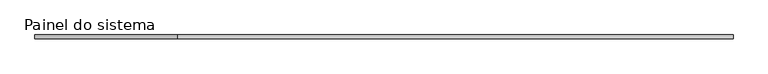
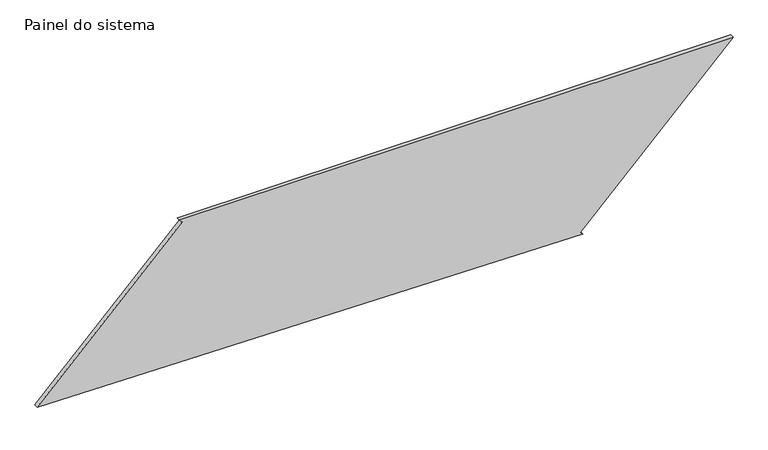
"""IFC4 building model written with IfcOpenShell, lengths in millimetres: plate geometry, Painel do sistema : Envidraçado."""

from ifc_helpers import new_model, si_unit, frame, origin, place, context, project, spatial, polyline, outline, extrude, source, transform, mapped, element, save


def painel_do_sistema_c34546bd(model_context):
    return source(origin(), model_context, "Body", "SweptSolid", [
        extrude(outline(polyline([(0.0, 1285.1979047), (17.655268, 1267.4978621), (1013.8299287, 2261.1525654), (1013.8299287, -1337.1847179), (996.1746607, -1319.4846752), (52.1186543, -2261.1525654), (0.0, 1285.1979047)])), frame((0.0, 24.5, 0.0), z_axis=(0.0, 1.0, 0.0), x_axis=(0.0, 0.0, 1.0)), (0.0, 0.0, 1.0), 25.0),
    ])


if __name__ == "__main__":
    model = new_model("IFC4")
    model_context = context("Model", 3, world=origin())
    ifc_project = project(units=[si_unit("LENGTHUNIT", "METRE", prefix="MILLI")], contexts=[model_context])
    site = spatial("IfcSite", under=ifc_project)
    building = spatial("IfcBuilding", under=site)
    placement = place(None, origin())
    painel_do_sistema_shape = painel_do_sistema_c34546bd(model_context)
    element("IfcPlate", 1, ObjectType="Painel do sistema : Envidraçado", at=placement, inside=building, context=model_context, shape_type="MappedRepresentation", body=[
        mapped(painel_do_sistema_shape, transform((0.0, 0.0, 0.0), x_axis=(1.0, 0.0, 0.0), y_axis=(0.0, 1.0, 0.0), z_axis=(0.0, 0.0, 1.0))),
    ])
    save(model, "model.ifc")

# Revit data of these elements
# Type "Painel do sistema : Envidraçado"
#   Construction Type Id = "GSP4R"
#   Analytic Construction = "Vidraça única Pilkington 1/8 pol"
#   Visual Light Transmittance = 0.9
#   Solar Heat Gain Coefficient = 0.86
#   Heat Transfer Coefficient (U) = 6.7069 W/(m²·K)
# Element 1 (IfcPlate, "Painel do sistema : Envidraçado")
#   Materials on its faces: "Vidro"
# Materials
#   "Vidro": class "Vidro", colour RGB 0 128 192, transparency 0.9, Description = "Vidro de sílica", Cost = 0
